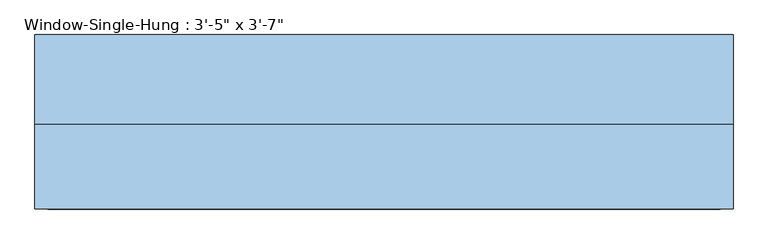
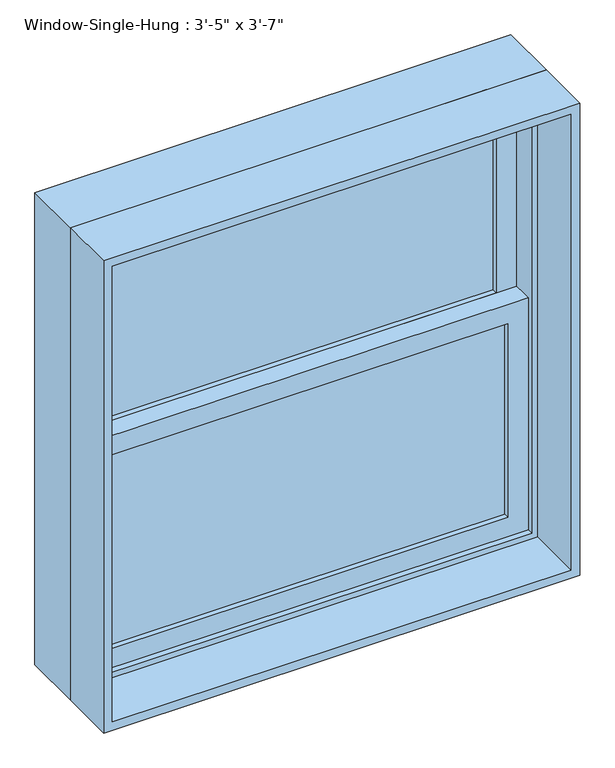
"""IFC4 building model written with IfcOpenShell, lengths in millimetres: window geometry."""

from ifc_helpers import new_model, si_unit, frame, origin, place, context, project, spatial, polyline, outline, extrude, source, transform, mapped, element, save


def window_d175fa0a(model_context):
    return source(origin(), model_context, "Body", "SweptSolid", [
        extrude(outline(polyline([(444.5, 50.8), (444.5, 44.45), (-444.5, 44.45), (-444.5, 50.8), (444.5, 50.8)])), frame((0.0, 0.0, 990.6), z_axis=(0.0, 0.0, 1.0), x_axis=(1.0, 0.0, 0.0)), (0.0, 0.0, 1.0), 447.675),
        extrude(outline(polyline([(-444.5, 38.1), (444.5, 38.1), (444.5, 31.75), (-444.5, 31.75), (-444.5, 38.1)])), frame((0.0, 0.0, 990.6), z_axis=(0.0, 0.0, 1.0), x_axis=(1.0, 0.0, 0.0)), (0.0, 0.0, 1.0), 447.675),
        extrude(outline(polyline([(444.5, 95.25), (444.5, 88.9), (-444.5, 88.9), (-444.5, 95.25), (444.5, 95.25)])), frame((0.0, 0.0, 1482.725), z_axis=(0.0, 0.0, 1.0), x_axis=(1.0, 0.0, 0.0)), (0.0, 0.0, 1.0), 447.675),
        extrude(outline(polyline([(-444.5, 82.55), (444.5, 82.55), (444.5, 76.2), (-444.5, 76.2), (-444.5, 82.55)])), frame((0.0, 0.0, 1482.725), z_axis=(0.0, 0.0, 1.0), x_axis=(1.0, 0.0, 0.0)), (0.0, 0.0, 1.0), 447.675),
        extrude(outline(polyline([(1482.725, -488.95), (946.15, -488.95), (946.15, 488.95), (1482.725, 488.95), (1482.725, -488.95)]), holes=[polyline([(1438.275, 444.5), (990.6, 444.5), (990.6, -444.5), (1438.275, -444.5), (1438.275, 444.5)])]), frame((0.0, 19.05, 0.0), z_axis=(0.0, 1.0, 0.0), x_axis=(0.0, 0.0, 1.0)), (0.0, 0.0, 1.0), 44.45),
        extrude(outline(polyline([(1974.85, -488.95), (1438.275, -488.95), (1438.275, 488.95), (1974.85, 488.95), (1974.85, -488.95)]), holes=[polyline([(1930.4, 444.5), (1482.725, 444.5), (1482.725, -444.5), (1930.4, -444.5), (1930.4, 444.5)])]), frame((0.0, 63.5, 0.0), z_axis=(0.0, 1.0, 0.0), x_axis=(0.0, 0.0, 1.0)), (0.0, 0.0, 1.0), 44.45),
        extrude(outline(polyline([(2006.6, -520.7), (914.4, -520.7), (914.4, 520.7), (2006.6, 520.7), (2006.6, -520.7)]), holes=[polyline([(1974.85, 488.95), (946.15, 488.95), (946.15, -488.95), (1974.85, -488.95), (1974.85, 488.95)])]), frame((0.0, 6.35, 0.0), z_axis=(0.0, 1.0, 0.0), x_axis=(0.0, 0.0, 1.0)), (0.0, 0.0, 1.0), 133.35),
        extrude(outline(polyline([(2006.6, 520.7), (2006.6, -520.7), (914.4, -520.7), (914.4, 520.7), (2006.6, 520.7)]), holes=[polyline([(1987.55, 501.65), (933.45, 501.65), (933.45, -501.65), (1987.55, -501.65), (1987.55, 501.65)])]), frame((0.0, -120.65, 0.0), z_axis=(0.0, 1.0, 0.0), x_axis=(0.0, 0.0, 1.0)), (0.0, 0.0, 1.0), 127.0),
    ])


if __name__ == "__main__":
    model = new_model("IFC4")
    model_context = context("Model", 3, world=origin())
    ifc_project = project(units=[si_unit("LENGTHUNIT", "METRE", prefix="MILLI")], contexts=[model_context])
    site = spatial("IfcSite", under=ifc_project)
    building = spatial("IfcBuilding", under=site)
    placement = place(None, origin())
    window_shape = window_d175fa0a(model_context)
    element("IfcWindow", 1, ObjectType="Window-Single-Hung : 3'-5\" x 3'-7\"", at=placement, inside=building, context=model_context, shape_type="MappedRepresentation", body=[
        mapped(window_shape, transform((0.0, 0.0, 0.0), x_axis=(1.0, 0.0, 0.0), y_axis=(0.0, 1.0, 0.0), z_axis=(0.0, 0.0, 1.0))),
    ])
    save(model, "model.ifc")

# Revit data of these elements
# Type "Window-Single-Hung : 3'-5\" x 3'-7\""
#   Type Mark = "07"
#   Fire Rating = "0.5h"
#   Construction Type Id = "DG-DR"
#   Assembly Code = "B2020100"
#   Analytic Construction = "Double glazing - domestic"
#   Wall Thickness [instance default] = 0' - 6"
#   Window Inset [instance default] = 0' - 0"
#   Visual Light Transmittance = 0.81
#   Thermal Resistance (R) = 0.319569 (m²·K)/W
#   Solar Heat Gain Coefficient = 0.76
#   Muntin Width = 2' - 11"
#   Muntin Height = 1' - 5 5/8"
#   Interior Wall Closure [instance default] = 0' - 1 1/2"
#   Rough Width = 3' - 5 1/2"
#   Rough Height = 3' - 7 1/2"
#   Frame Extension [instance default] = 0' - 1 1/4"
#   Exterior Wall Closure [instance default] = 0' - 0 1/2"
#   Extension Jamb [instance default] = 0' - 1 1/2"
#   Heat Transfer Coefficient (U) = 3.12929 W/(m²·K)
#   Height = 3' - 7"
#   Width = 3' - 5"
#   Top Muntin Visibility = no
#   Indicator Visibility = no
#   Extension Jamb Visibility [instance default] = yes
#   Interior Trim Visibility [instance default] = yes
#   Exterior Trim Visibility [instance default] = yes
#   Bottom Muntin Visibility = no
#   Muntin Pattern = Muntin Pattern_2x2 : Muntin Pattern_2x2
#   Interior Trim Material = 1X WOOD COMPOSITE TRIM
#   Interior Trim = Trim-Window-Interior-Flat : Picture Frame
#   Exterior Trim Material = 1X WOOD COMPOSITE TRIM
#   Exterior Trim = Trim-Window-Exterior-Flat : with Sill
#   Glass Panel Material = NEW DOUBLE HUNG WINDOWS (TYP.)
#   Exterior Frame Material = 1X WOOD COMPOSITE TRIM
#   Interior Frame Material = 1X WOOD COMPOSITE TRIM
#   Wall Closure = (empty or 0)
# Element 1 (IfcWindow, "Window-Single-Hung : 3'-5\" x 3'-7\"")
#   Wall Thickness = 0' - 9 1/2"
#   Extension Jamb = 0' - 5"
#   Materials on its faces: "1X WOOD COMPOSITE TRIM", "NEW DOUBLE HUNG WINDOWS (TYP.)"
# Materials
#   "1X WOOD COMPOSITE TRIM": class "Generic", colour RGB 88 61 61, transparency 0, Cost = 0
#   "NEW DOUBLE HUNG WINDOWS (TYP.)": class "Glass", colour RGB 218 227 224, transparency 0.85, Description = "Soda Lime Glass", Cost = 0
